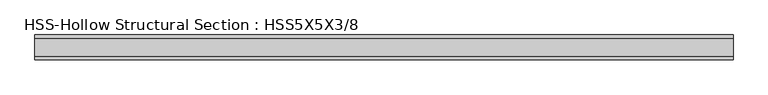
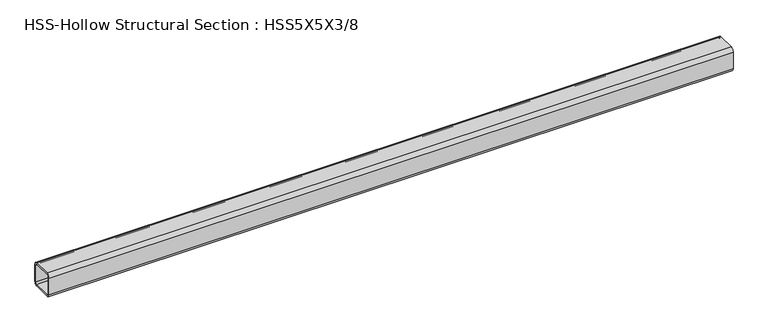
"""IFC4 building model written with IfcOpenShell, lengths in millimetres: member geometry, HSS-Hollow Structural Section : HSS5X5X3/8."""

from ifc_helpers import new_model, si_unit, point, frame, frame_2d, origin, place, context, project, spatial, polyline, circle_curve, trimmed, segment, composite_curve, outline, extrude, source, transform, mapped, element, save


def hss_hollow_structural_section_hss5x5x3_8_f1e67e1b(model_context):
    return source(origin(), model_context, "Body", "SweptSolid", [
        extrude(outline(composite_curve([segment(polyline([(63.5, 45.7708), (63.5, -45.7708)]), True, "CONTINUOUS"), segment(trimmed(circle_curve(frame_2d((45.7708, -45.7708)), 17.7292), [point((63.5, -45.7708))], [point((45.7708, -63.5))], False, "CARTESIAN"), True, "CONTINUOUS"), segment(polyline([(45.7708, -63.5), (-45.7708, -63.5)]), True, "CONTINUOUS"), segment(trimmed(circle_curve(frame_2d((-45.7708, -45.7708)), 17.7292), [point((-45.7708, -63.5))], [point((-63.5, -45.7708))], False, "CARTESIAN"), True, "CONTINUOUS"), segment(polyline([(-63.5, -45.7708), (-63.5, 45.7708)]), True, "CONTINUOUS"), segment(trimmed(circle_curve(frame_2d((-45.7708, 45.7708)), 17.7292), [point((-63.5, 45.7708))], [point((-45.7708, 63.5))], False, "CARTESIAN"), True, "CONTINUOUS"), segment(polyline([(-45.7708, 63.5), (45.7708, 63.5)]), True, "CONTINUOUS"), segment(trimmed(circle_curve(frame_2d((45.7708, 45.7708)), 17.7292), [point((45.7708, 63.5))], [point((63.5, 45.7708))], False, "CARTESIAN"), True, "CONTINUOUS")], self_intersect=False), holes=[composite_curve([segment(trimmed(circle_curve(frame_2d((-45.7708, 45.7708)), 8.8646), [point((-45.7708, 54.6354))], [point((-54.6354, 45.7708))], True, "CARTESIAN"), True, "CONTINUOUS"), segment(polyline([(-54.6354, 45.7708), (-54.6354, -45.7708)]), True, "CONTINUOUS"), segment(trimmed(circle_curve(frame_2d((-45.7708, -45.7708)), 8.8646), [point((-54.6354, -45.7708))], [point((-45.7708, -54.6354))], True, "CARTESIAN"), True, "CONTINUOUS"), segment(polyline([(-45.7708, -54.6354), (45.7708, -54.6354)]), True, "CONTINUOUS"), segment(trimmed(circle_curve(frame_2d((45.7708, -45.7708)), 8.8646), [point((45.7708, -54.6354))], [point((54.6354, -45.7708))], True, "CARTESIAN"), True, "CONTINUOUS"), segment(polyline([(54.6354, -45.7708), (54.6354, 45.7708)]), True, "CONTINUOUS"), segment(trimmed(circle_curve(frame_2d((45.7708, 45.7708)), 8.8646), [point((54.6354, 45.7708))], [point((45.7708, 54.6354))], True, "CARTESIAN"), True, "CONTINUOUS"), segment(polyline([(45.7708, 54.6354), (-45.7708, 54.6354)]), True, "CONTINUOUS")], self_intersect=False)]), frame((-1783.2627481, 0.0, 0.0), z_axis=(1.0, 0.0, 0.0), x_axis=(0.0, 1.0, 0.0)), (0.0, 0.0, 1.0), 3566.5254963),
    ])


if __name__ == "__main__":
    model = new_model("IFC4")
    model_context = context("Model", 3, world=origin())
    ifc_project = project(units=[si_unit("LENGTHUNIT", "METRE", prefix="MILLI")], contexts=[model_context])
    site = spatial("IfcSite", under=ifc_project)
    building = spatial("IfcBuilding", under=site)
    placement = place(None, origin())
    hss_hollow_structural_section_hss5x5x3_8_shape = hss_hollow_structural_section_hss5x5x3_8_f1e67e1b(model_context)
    element("IfcMember", 1, ObjectType="HSS-Hollow Structural Section : HSS5X5X3/8", at=placement, inside=building, context=model_context, shape_type="MappedRepresentation", body=[
        mapped(hss_hollow_structural_section_hss5x5x3_8_shape, transform((0.0, 0.0, 0.0), x_axis=(1.0, 0.0, 0.0), y_axis=(0.0, 1.0, 0.0), z_axis=(0.0, 0.0, 1.0))),
    ])
    save(model, "model.ifc")

# Revit data of these elements
# Type "HSS-Hollow Structural Section : HSS5X5X3/8"
#   Assembly Code = "B10"
#   Shape = "Square"
#   W = 22.3
#   Ht = 0' - 5"
#   Length [instance default] = 5' - 0"
#   b = 0' - 5"
#   kr = 0' - 0.698"
#   t = 0' - 0.349"
#   A = 0.0429167 SF
#   Structural Material [instance default] = Steel ASTM A500, Grade B, Rectangular and Square
# Element 1 (IfcMember, "HSS-Hollow Structural Section : HSS5X5X3/8")
#   Materials on its faces: "Steel ASTM A500, Grade B, Rectangular and Square"
# Materials
#   "Steel ASTM A500, Grade B, Rectangular and Square": class "Metal", colour RGB 199 199 199, transparency 0, Description = "Carbon steel", Cost = 0
